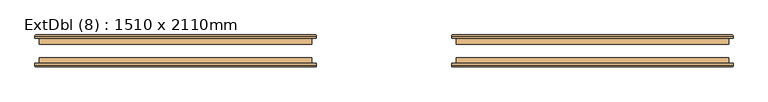
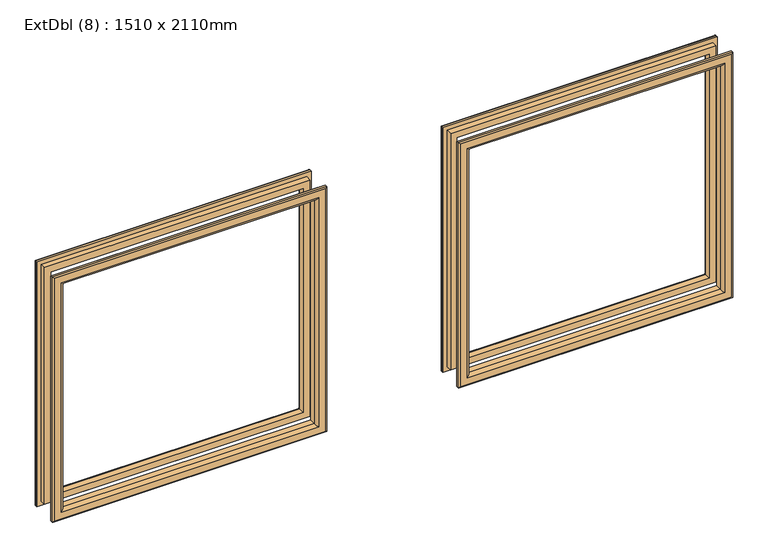
"""IFC4 building model written with IfcOpenShell, lengths in millimetres: door geometry, ExtDbl (8) : 1510 x 2110mm."""

from ifc_helpers import new_model, si_unit, frame, origin, place, context, project, spatial, ellipse_curve, source, transform, mapped, element, save
from ifc_brep_helpers import plane_surface, cylinder_surface, advanced_brep


def extdbl_8_1510_x_2110mm_bd11c51c(model_context):
    return source(origin(), model_context, "Body", "AdvancedBrep", [
        advanced_brep(
        [(-126.5, 31.0, 808.5), (-126.5, 21.0, 808.5), (-126.5, 21.0, 358.5), (-126.5, 31.0, 358.5), (-138.5, 20.0, 796.5), (-138.5, 31.0, 796.5), (-138.5, 31.0, 370.5), (-138.5, 20.0, 370.5), (-133.5, 15.0, 801.5), (-133.5, 15.0, 365.5), (-118.5, 17.0, 816.5), (-120.5, 15.0, 814.5), (-120.5, 15.0, 352.5), (-118.5, 17.0, 350.5), (-118.5, 21.0, 816.5), (-118.5, 21.0, 350.5), (-603.5, 21.0, 358.5), (-603.5, 31.0, 358.5), (-591.5, 31.0, 370.5), (-591.5, 20.0, 370.5), (-596.5, 15.0, 365.5), (-609.5, 15.0, 352.5), (-611.5, 17.0, 350.5), (-611.5, 21.0, 350.5), (-603.5, 21.0, 808.5), (-603.5, 31.0, 808.5), (-591.5, 31.0, 796.5), (-591.5, 20.0, 796.5), (-596.5, 15.0, 801.5), (-609.5, 15.0, 814.5), (-611.5, 17.0, 816.5), (-611.5, 21.0, 816.5)],
        [
            (0, 1),
            (1, 2),
            (2, 3),
            (3, 0),
            (4, 5),
            (5, 6),
            (6, 7),
            (7, 4),
            (8, 4, ellipse_curve(frame((-133.5, 20.0, 801.5), z_axis=(0.707106781186552, 0.0, -0.7071067811865429), x_axis=(0.7071067811865428, 0.0, 0.7071067811865521)), 7.0710678, 5.0)),
            (7, 9, ellipse_curve(frame((-133.5, 20.0, 365.5), z_axis=(0.7071067811865429, 0.0, 0.707106781186552), x_axis=(-0.707106781186552, 0.0, 0.707106781186543)), 7.0710678, 5.0)),
            (9, 8),
            (10, 11, ellipse_curve(frame((-120.5, 17.0, 814.5), z_axis=(0.707106781186552, 0.0, -0.7071067811865429), x_axis=(0.7071067811865428, 0.0, 0.7071067811865521)), 2.8284271, 2.0)),
            (11, 12),
            (12, 13, ellipse_curve(frame((-120.5, 17.0, 352.5), z_axis=(0.7071067811865429, 0.0, 0.707106781186552), x_axis=(-0.707106781186552, 0.0, 0.707106781186543)), 2.8284271, 2.0)),
            (13, 10),
            (14, 10),
            (13, 15),
            (15, 14),
            (2, 16),
            (16, 17),
            (17, 3),
            (6, 18),
            (18, 19),
            (19, 7),
            (19, 20, ellipse_curve(frame((-596.5, 20.0, 365.5), z_axis=(0.7071067811865521, 0.0, -0.7071067811865428), x_axis=(0.7071067811865429, 0.0, 0.707106781186552)), 7.0710678, 5.0)),
            (20, 9),
            (12, 21),
            (21, 22, ellipse_curve(frame((-609.5, 17.0, 352.5), z_axis=(0.7071067811865521, 0.0, -0.7071067811865428), x_axis=(0.7071067811865429, 0.0, 0.707106781186552)), 2.8284271, 2.0)),
            (22, 13),
            (22, 23),
            (23, 15),
            (16, 24),
            (24, 25),
            (25, 17),
            (18, 26),
            (26, 27),
            (27, 19),
            (27, 28, ellipse_curve(frame((-596.5, 20.0, 801.5), z_axis=(-0.7071067811865428, 0.0, -0.7071067811865521), x_axis=(0.707106781186552, 0.0, -0.7071067811865429)), 7.0710678, 5.0)),
            (28, 20),
            (21, 29),
            (29, 30, ellipse_curve(frame((-609.5, 17.0, 814.5), z_axis=(-0.7071067811865428, 0.0, -0.7071067811865521), x_axis=(0.707106781186552, 0.0, -0.7071067811865429)), 2.8284271, 2.0)),
            (30, 22),
            (30, 31),
            (31, 23),
            (31, 14),
            (1, 24),
            (0, 25),
            (5, 26),
            (4, 27),
            (8, 28),
            (11, 29),
            (10, 30),
        ],
        [
            plane_surface(frame((-126.5, 21.0, 808.5), z_axis=(1.0, 0.0, 0.0), x_axis=(0.0, 0.0, -1.0))),
            plane_surface(frame((-138.5, 31.0, 796.5), z_axis=(-1.0, 0.0, 0.0), x_axis=(0.0, 0.0, -1.0))),
            cylinder_surface(frame((-133.5, 20.0, 808.5), z_axis=(0.0, 0.0, 1.0), x_axis=(1.0, 0.0, 0.0)), 5.0),
            cylinder_surface(frame((-120.5, 17.0, 808.5), z_axis=(0.0, 0.0, 1.0), x_axis=(1.0, 0.0, 0.0)), 2.0),
            plane_surface(frame((-118.5, 17.0, 816.5), z_axis=(1.0, 0.0, 0.0), x_axis=(0.0, 0.0, -1.0))),
            plane_surface(frame((-126.5, 21.0, 358.5), z_axis=(0.0, 0.0, -1.0), x_axis=(-1.0, 0.0, 0.0))),
            plane_surface(frame((-138.5, 31.0, 370.5), z_axis=(0.0, 0.0, 1.0), x_axis=(-1.0, 0.0, 0.0))),
            cylinder_surface(frame((-126.5, 20.0, 365.5), z_axis=(1.0, 0.0, 0.0), x_axis=(0.0, 0.0, -1.0)), 5.0),
            cylinder_surface(frame((-126.5, 17.0, 352.5), z_axis=(1.0, 0.0, 0.0), x_axis=(0.0, 0.0, -1.0)), 2.0),
            plane_surface(frame((-118.5, 17.0, 350.5), z_axis=(0.0, 0.0, -1.0), x_axis=(-1.0, 0.0, 0.0))),
            plane_surface(frame((-603.5, 21.0, 358.5), z_axis=(-1.0, 0.0, 0.0), x_axis=(0.0, 0.0, 1.0))),
            plane_surface(frame((-591.5, 31.0, 370.5), z_axis=(1.0, 0.0, 0.0), x_axis=(0.0, 0.0, 1.0))),
            cylinder_surface(frame((-596.5, 20.0, 358.5), z_axis=(0.0, 0.0, -1.0), x_axis=(-1.0, 0.0, 0.0)), 5.0),
            cylinder_surface(frame((-609.5, 17.0, 358.5), z_axis=(0.0, 0.0, -1.0), x_axis=(-1.0, 0.0, 0.0)), 2.0),
            plane_surface(frame((-611.5, 17.0, 350.5), z_axis=(-1.0, 0.0, 0.0), x_axis=(0.0, 0.0, 1.0))),
            plane_surface(frame((-611.5, 21.0, 816.5), z_axis=(0.0, 1.0, 0.0), x_axis=(1.0, 0.0, 0.0))),
            plane_surface(frame((-603.5, 21.0, 808.5), z_axis=(0.0, 0.0, 1.0), x_axis=(1.0, 0.0, 0.0))),
            plane_surface(frame((-603.5, 31.0, 808.5), z_axis=(0.0, 1.0, 0.0), x_axis=(1.0, 0.0, 0.0))),
            plane_surface(frame((-591.5, 31.0, 796.5), z_axis=(0.0, 0.0, -1.0), x_axis=(1.0, 0.0, 0.0))),
            cylinder_surface(frame((-603.5, 20.0, 801.5), z_axis=(-1.0, 0.0, 0.0), x_axis=(0.0, 0.0, 1.0)), 5.0),
            plane_surface(frame((-596.5, 15.0, 801.5), z_axis=(0.0, -1.0, 0.0), x_axis=(1.0, 0.0, 0.0))),
            cylinder_surface(frame((-603.5, 17.0, 814.5), z_axis=(-1.0, 0.0, 0.0), x_axis=(0.0, 0.0, 1.0)), 2.0),
            plane_surface(frame((-611.5, 17.0, 816.5), z_axis=(0.0, 0.0, 1.0), x_axis=(1.0, 0.0, 0.0))),
        ],
        [
            (0, [[1, 2, 3, 4]]),
            (1, [[5, 6, 7, 8]]),
            (2, [[9, -8, 10, 11]]),
            (3, [[12, 13, 14, 15]]),
            (4, [[16, -15, 17, 18]]),
            (5, [[-3, 19, 20, 21]]),
            (6, [[-7, 22, 23, 24]]),
            (7, [[-10, -24, 25, 26]]),
            (8, [[-14, 27, 28, 29]]),
            (9, [[-17, -29, 30, 31]]),
            (10, [[-20, 32, 33, 34]]),
            (11, [[-23, 35, 36, 37]]),
            (12, [[-25, -37, 38, 39]]),
            (13, [[-28, 40, 41, 42]]),
            (14, [[-30, -42, 43, 44]]),
            (15, [[-31, -44, 45, -18], [46, -32, -19, -2]]),
            (16, [[-33, -46, -1, 47]]),
            (17, [[-21, -34, -47, -4], [48, -35, -22, -6]]),
            (18, [[-36, -48, -5, 49]]),
            (19, [[-38, -49, -9, 50]]),
            (20, [[51, -40, -27, -13], [-26, -39, -50, -11]]),
            (21, [[-41, -51, -12, 52]]),
            (22, [[-43, -52, -16, -45]]),
        ],
    ),
        advanced_brep(
        [(-603.5, 55.0, 808.5), (-603.5, 65.0, 808.5), (-603.5, 65.0, 358.5), (-603.5, 55.0, 358.5), (-591.5, 66.0, 796.5), (-591.5, 55.0, 796.5), (-591.5, 55.0, 370.5), (-591.5, 66.0, 370.5), (-596.5, 71.0, 801.5), (-596.5, 71.0, 365.5), (-611.5, 69.0, 816.5), (-609.5, 71.0, 814.5), (-609.5, 71.0, 352.5), (-611.5, 69.0, 350.5), (-611.5, 65.0, 816.5), (-611.5, 65.0, 350.5), (-126.5, 65.0, 358.5), (-126.5, 55.0, 358.5), (-138.5, 55.0, 370.5), (-138.5, 66.0, 370.5), (-133.5, 71.0, 365.5), (-120.5, 71.0, 352.5), (-118.5, 69.0, 350.5), (-118.5, 65.0, 350.5), (-126.5, 65.0, 808.5), (-126.5, 55.0, 808.5), (-138.5, 55.0, 796.5), (-138.5, 66.0, 796.5), (-133.5, 71.0, 801.5), (-120.5, 71.0, 814.5), (-118.5, 69.0, 816.5), (-118.5, 65.0, 816.5)],
        [
            (0, 1),
            (1, 2),
            (2, 3),
            (3, 0),
            (4, 5),
            (5, 6),
            (6, 7),
            (7, 4),
            (8, 4, ellipse_curve(frame((-596.5, 66.0, 801.5), z_axis=(-0.7071067811865477, 0.0, -0.7071067811865472), x_axis=(-0.7071067811865471, 0.0, 0.7071067811865478)), 7.0710678, 5.0)),
            (7, 9, ellipse_curve(frame((-596.5, 66.0, 365.5), z_axis=(-0.7071067811865472, 0.0, 0.7071067811865477), x_axis=(0.7071067811865476, 0.0, 0.7071067811865475)), 7.0710678, 5.0)),
            (9, 8),
            (10, 11, ellipse_curve(frame((-609.5, 69.0, 814.5), z_axis=(-0.7071067811865477, 0.0, -0.7071067811865472), x_axis=(-0.7071067811865471, 0.0, 0.7071067811865478)), 2.8284271, 2.0)),
            (11, 12),
            (12, 13, ellipse_curve(frame((-609.5, 69.0, 352.5), z_axis=(-0.7071067811865472, 0.0, 0.7071067811865477), x_axis=(0.7071067811865476, 0.0, 0.7071067811865475)), 2.8284271, 2.0)),
            (13, 10),
            (14, 10),
            (13, 15),
            (15, 14),
            (2, 16),
            (16, 17),
            (17, 3),
            (6, 18),
            (18, 19),
            (19, 7),
            (19, 20, ellipse_curve(frame((-133.5, 66.0, 365.5), z_axis=(-0.7071067811865477, 0.0, -0.7071067811865474), x_axis=(-0.7071067811865474, 0.0, 0.7071067811865478)), 7.0710678, 5.0)),
            (20, 9),
            (12, 21),
            (21, 22, ellipse_curve(frame((-120.5, 69.0, 352.5), z_axis=(-0.7071067811865477, 0.0, -0.7071067811865474), x_axis=(-0.7071067811865474, 0.0, 0.7071067811865478)), 2.8284271, 2.0)),
            (22, 13),
            (22, 23),
            (23, 15),
            (16, 24),
            (24, 25),
            (25, 17),
            (18, 26),
            (26, 27),
            (27, 19),
            (27, 28, ellipse_curve(frame((-133.5, 66.0, 801.5), z_axis=(0.7071067811865474, 0.0, -0.7071067811865478), x_axis=(-0.7071067811865479, 0.0, -0.7071067811865471)), 7.0710678, 5.0)),
            (28, 20),
            (21, 29),
            (29, 30, ellipse_curve(frame((-120.5, 69.0, 814.5), z_axis=(0.7071067811865474, 0.0, -0.7071067811865478), x_axis=(-0.7071067811865479, 0.0, -0.7071067811865471)), 2.8284271, 2.0)),
            (30, 22),
            (30, 31),
            (31, 23),
            (31, 14),
            (1, 24),
            (0, 25),
            (5, 26),
            (4, 27),
            (8, 28),
            (11, 29),
            (10, 30),
        ],
        [
            plane_surface(frame((-603.5, 65.0, 808.5), z_axis=(-1.0, 0.0, 0.0), x_axis=(0.0, 0.0, -1.0))),
            plane_surface(frame((-591.5, 55.0, 796.5), z_axis=(1.0, 0.0, 0.0), x_axis=(0.0, 0.0, -1.0))),
            cylinder_surface(frame((-596.5, 66.0, 808.5), z_axis=(0.0, 0.0, 1.0), x_axis=(-1.0, 0.0, 0.0)), 5.0),
            cylinder_surface(frame((-609.5, 69.0, 808.5), z_axis=(0.0, 0.0, 1.0), x_axis=(-1.0, 0.0, 0.0)), 2.0),
            plane_surface(frame((-611.5, 69.0, 816.5), z_axis=(-1.0, 0.0, 0.0), x_axis=(0.0, 0.0, -1.0))),
            plane_surface(frame((-603.5, 65.0, 358.5), z_axis=(0.0, 0.0, -1.0), x_axis=(1.0, 0.0, 0.0))),
            plane_surface(frame((-591.5, 55.0, 370.5), z_axis=(0.0, 0.0, 1.0), x_axis=(1.0, 0.0, 0.0))),
            cylinder_surface(frame((-603.5, 66.0, 365.5), z_axis=(-1.0, 0.0, 0.0), x_axis=(0.0, 0.0, -1.0)), 5.0),
            cylinder_surface(frame((-603.5, 69.0, 352.5), z_axis=(-1.0, 0.0, 0.0), x_axis=(0.0, 0.0, -1.0)), 2.0),
            plane_surface(frame((-611.5, 69.0, 350.5), z_axis=(0.0, 0.0, -1.0), x_axis=(1.0, 0.0, 0.0))),
            plane_surface(frame((-126.5, 65.0, 358.5), z_axis=(1.0, 0.0, 0.0), x_axis=(0.0, 0.0, 1.0))),
            plane_surface(frame((-138.5, 55.0, 370.5), z_axis=(-1.0, 0.0, 0.0), x_axis=(0.0, 0.0, 1.0))),
            cylinder_surface(frame((-133.5, 66.0, 358.5), z_axis=(0.0, 0.0, -1.0), x_axis=(1.0, 0.0, 0.0)), 5.0),
            cylinder_surface(frame((-120.5, 69.0, 358.5), z_axis=(0.0, 0.0, -1.0), x_axis=(1.0, 0.0, 0.0)), 2.0),
            plane_surface(frame((-118.5, 69.0, 350.5), z_axis=(1.0, 0.0, 0.0), x_axis=(0.0, 0.0, 1.0))),
            plane_surface(frame((-118.5, 65.0, 816.5), z_axis=(0.0, -1.0, 0.0), x_axis=(-1.0, 0.0, 0.0))),
            plane_surface(frame((-126.5, 65.0, 808.5), z_axis=(0.0, 0.0, 1.0), x_axis=(-1.0, 0.0, 0.0))),
            plane_surface(frame((-126.5, 55.0, 808.5), z_axis=(0.0, -1.0, 0.0), x_axis=(-1.0, 0.0, 0.0))),
            plane_surface(frame((-138.5, 55.0, 796.5), z_axis=(0.0, 0.0, -1.0), x_axis=(-1.0, 0.0, 0.0))),
            cylinder_surface(frame((-126.5, 66.0, 801.5), z_axis=(1.0, 0.0, 0.0), x_axis=(0.0, 0.0, 1.0)), 5.0),
            plane_surface(frame((-133.5, 71.0, 801.5), z_axis=(0.0, 1.0, 0.0), x_axis=(-1.0, 0.0, 0.0))),
            cylinder_surface(frame((-126.5, 69.0, 814.5), z_axis=(1.0, 0.0, 0.0), x_axis=(0.0, 0.0, 1.0)), 2.0),
            plane_surface(frame((-118.5, 69.0, 816.5), z_axis=(0.0, 0.0, 1.0), x_axis=(-1.0, 0.0, 0.0))),
        ],
        [
            (0, [[1, 2, 3, 4]]),
            (1, [[5, 6, 7, 8]]),
            (2, [[9, -8, 10, 11]]),
            (3, [[12, 13, 14, 15]]),
            (4, [[16, -15, 17, 18]]),
            (5, [[-3, 19, 20, 21]]),
            (6, [[-7, 22, 23, 24]]),
            (7, [[-10, -24, 25, 26]]),
            (8, [[-14, 27, 28, 29]]),
            (9, [[-17, -29, 30, 31]]),
            (10, [[-20, 32, 33, 34]]),
            (11, [[-23, 35, 36, 37]]),
            (12, [[-25, -37, 38, 39]]),
            (13, [[-28, 40, 41, 42]]),
            (14, [[-30, -42, 43, 44]]),
            (15, [[-31, -44, 45, -18], [46, -32, -19, -2]]),
            (16, [[-33, -46, -1, 47]]),
            (17, [[-21, -34, -47, -4], [48, -35, -22, -6]]),
            (18, [[-36, -48, -5, 49]]),
            (19, [[-38, -49, -9, 50]]),
            (20, [[51, -40, -27, -13], [-26, -39, -50, -11]]),
            (21, [[-41, -51, -12, 52]]),
            (22, [[-43, -52, -16, -45]]),
        ],
    ),
        advanced_brep(
        [(603.5, 31.0, 808.5), (603.5, 21.0, 808.5), (603.5, 21.0, 358.5), (603.5, 31.0, 358.5), (591.5, 20.0, 796.5), (591.5, 31.0, 796.5), (591.5, 31.0, 370.5), (591.5, 20.0, 370.5), (596.5, 15.0, 801.5), (596.5, 15.0, 365.5), (611.5, 17.0, 816.5), (609.5, 15.0, 814.5), (609.5, 15.0, 352.5), (611.5, 17.0, 350.5), (611.5, 21.0, 816.5), (611.5, 21.0, 350.5), (126.5, 21.0, 358.5), (126.5, 31.0, 358.5), (138.5, 31.0, 370.5), (138.5, 20.0, 370.5), (133.5, 15.0, 365.5), (120.5, 15.0, 352.5), (118.5, 17.0, 350.5), (118.5, 21.0, 350.5), (126.5, 21.0, 808.5), (126.5, 31.0, 808.5), (138.5, 31.0, 796.5), (138.5, 20.0, 796.5), (133.5, 15.0, 801.5), (120.5, 15.0, 814.5), (118.5, 17.0, 816.5), (118.5, 21.0, 816.5)],
        [
            (0, 1),
            (1, 2),
            (2, 3),
            (3, 0),
            (4, 5),
            (5, 6),
            (6, 7),
            (7, 4),
            (8, 4, ellipse_curve(frame((596.5, 20.0, 801.5), z_axis=(0.7071067811865519, 0.0, -0.707106781186543), x_axis=(0.7071067811865429, 0.0, 0.7071067811865521)), 7.0710678, 5.0)),
            (7, 9, ellipse_curve(frame((596.5, 20.0, 365.5), z_axis=(0.707106781186543, 0.0, 0.707106781186552), x_axis=(-0.707106781186552, 0.0, 0.707106781186543)), 7.0710678, 5.0)),
            (9, 8),
            (10, 11, ellipse_curve(frame((609.5, 17.0, 814.5), z_axis=(0.7071067811865519, 0.0, -0.707106781186543), x_axis=(0.7071067811865429, 0.0, 0.7071067811865521)), 2.8284271, 2.0)),
            (11, 12),
            (12, 13, ellipse_curve(frame((609.5, 17.0, 352.5), z_axis=(0.707106781186543, 0.0, 0.707106781186552), x_axis=(-0.707106781186552, 0.0, 0.707106781186543)), 2.8284271, 2.0)),
            (13, 10),
            (14, 10),
            (13, 15),
            (15, 14),
            (2, 16),
            (16, 17),
            (17, 3),
            (6, 18),
            (18, 19),
            (19, 7),
            (19, 20, ellipse_curve(frame((133.5, 20.0, 365.5), z_axis=(0.707106781186552, 0.0, -0.707106781186543), x_axis=(0.7071067811865429, 0.0, 0.707106781186552)), 7.0710678, 5.0)),
            (20, 9),
            (12, 21),
            (21, 22, ellipse_curve(frame((120.5, 17.0, 352.5), z_axis=(0.707106781186552, 0.0, -0.707106781186543), x_axis=(0.7071067811865429, 0.0, 0.707106781186552)), 2.8284271, 2.0)),
            (22, 13),
            (22, 23),
            (23, 15),
            (16, 24),
            (24, 25),
            (25, 17),
            (18, 26),
            (26, 27),
            (27, 19),
            (27, 28, ellipse_curve(frame((133.5, 20.0, 801.5), z_axis=(-0.7071067811865431, 0.0, -0.707106781186552), x_axis=(0.7071067811865521, 0.0, -0.7071067811865429)), 7.0710678, 5.0)),
            (28, 20),
            (21, 29),
            (29, 30, ellipse_curve(frame((120.5, 17.0, 814.5), z_axis=(-0.7071067811865431, 0.0, -0.707106781186552), x_axis=(0.7071067811865521, 0.0, -0.7071067811865429)), 2.8284271, 2.0)),
            (30, 22),
            (30, 31),
            (31, 23),
            (31, 14),
            (1, 24),
            (0, 25),
            (5, 26),
            (4, 27),
            (8, 28),
            (11, 29),
            (10, 30),
        ],
        [
            plane_surface(frame((603.5, 21.0, 808.5), z_axis=(1.0, 0.0, 0.0), x_axis=(0.0, 0.0, -1.0))),
            plane_surface(frame((591.5, 31.0, 796.5), z_axis=(-1.0, 0.0, 0.0), x_axis=(0.0, 0.0, -1.0))),
            cylinder_surface(frame((596.5, 20.0, 808.5), z_axis=(0.0, 0.0, 1.0), x_axis=(1.0, 0.0, 0.0)), 5.0),
            cylinder_surface(frame((609.5, 17.0, 808.5), z_axis=(0.0, 0.0, 1.0), x_axis=(1.0, 0.0, 0.0)), 2.0),
            plane_surface(frame((611.5, 17.0, 816.5), z_axis=(1.0, 0.0, 0.0), x_axis=(0.0, 0.0, -1.0))),
            plane_surface(frame((603.5, 21.0, 358.5), z_axis=(0.0, 0.0, -1.0), x_axis=(-1.0, 0.0, 0.0))),
            plane_surface(frame((591.5, 31.0, 370.5), z_axis=(0.0, 0.0, 1.0), x_axis=(-1.0, 0.0, 0.0))),
            cylinder_surface(frame((603.5, 20.0, 365.5), z_axis=(1.0, 0.0, 0.0), x_axis=(0.0, 0.0, -1.0)), 5.0),
            cylinder_surface(frame((603.5, 17.0, 352.5), z_axis=(1.0, 0.0, 0.0), x_axis=(0.0, 0.0, -1.0)), 2.0),
            plane_surface(frame((611.5, 17.0, 350.5), z_axis=(0.0, 0.0, -1.0), x_axis=(-1.0, 0.0, 0.0))),
            plane_surface(frame((126.5, 21.0, 358.5), z_axis=(-1.0, 0.0, 0.0), x_axis=(0.0, 0.0, 1.0))),
            plane_surface(frame((138.5, 31.0, 370.5), z_axis=(1.0, 0.0, 0.0), x_axis=(0.0, 0.0, 1.0))),
            cylinder_surface(frame((133.5, 20.0, 358.5), z_axis=(0.0, 0.0, -1.0), x_axis=(-1.0, 0.0, 0.0)), 5.0),
            cylinder_surface(frame((120.5, 17.0, 358.5), z_axis=(0.0, 0.0, -1.0), x_axis=(-1.0, 0.0, 0.0)), 2.0),
            plane_surface(frame((118.5, 17.0, 350.5), z_axis=(-1.0, 0.0, 0.0), x_axis=(0.0, 0.0, 1.0))),
            plane_surface(frame((118.5, 21.0, 816.5), z_axis=(0.0, 1.0, 0.0), x_axis=(1.0, 0.0, 0.0))),
            plane_surface(frame((126.5, 21.0, 808.5), z_axis=(0.0, 0.0, 1.0), x_axis=(1.0, 0.0, 0.0))),
            plane_surface(frame((126.5, 31.0, 808.5), z_axis=(0.0, 1.0, 0.0), x_axis=(1.0, 0.0, 0.0))),
            plane_surface(frame((138.5, 31.0, 796.5), z_axis=(0.0, 0.0, -1.0), x_axis=(1.0, 0.0, 0.0))),
            cylinder_surface(frame((126.5, 20.0, 801.5), z_axis=(-1.0, 0.0, 0.0), x_axis=(0.0, 0.0, 1.0)), 5.0),
            plane_surface(frame((133.5, 15.0, 801.5), z_axis=(0.0, -1.0, 0.0), x_axis=(1.0, 0.0, 0.0))),
            cylinder_surface(frame((126.5, 17.0, 814.5), z_axis=(-1.0, 0.0, 0.0), x_axis=(0.0, 0.0, 1.0)), 2.0),
            plane_surface(frame((118.5, 17.0, 816.5), z_axis=(0.0, 0.0, 1.0), x_axis=(1.0, 0.0, 0.0))),
        ],
        [
            (0, [[1, 2, 3, 4]]),
            (1, [[5, 6, 7, 8]]),
            (2, [[9, -8, 10, 11]]),
            (3, [[12, 13, 14, 15]]),
            (4, [[16, -15, 17, 18]]),
            (5, [[-3, 19, 20, 21]]),
            (6, [[-7, 22, 23, 24]]),
            (7, [[-10, -24, 25, 26]]),
            (8, [[-14, 27, 28, 29]]),
            (9, [[-17, -29, 30, 31]]),
            (10, [[-20, 32, 33, 34]]),
            (11, [[-23, 35, 36, 37]]),
            (12, [[-25, -37, 38, 39]]),
            (13, [[-28, 40, 41, 42]]),
            (14, [[-30, -42, 43, 44]]),
            (15, [[-31, -44, 45, -18], [46, -32, -19, -2]]),
            (16, [[-33, -46, -1, 47]]),
            (17, [[-21, -34, -47, -4], [48, -35, -22, -6]]),
            (18, [[-36, -48, -5, 49]]),
            (19, [[-38, -49, -9, 50]]),
            (20, [[51, -40, -27, -13], [-26, -39, -50, -11]]),
            (21, [[-41, -51, -12, 52]]),
            (22, [[-43, -52, -16, -45]]),
        ],
    ),
        advanced_brep(
        [(126.5, 55.0, 808.5), (126.5, 65.0, 808.5), (126.5, 65.0, 358.5), (126.5, 55.0, 358.5), (138.5, 66.0, 796.5), (138.5, 55.0, 796.5), (138.5, 55.0, 370.5), (138.5, 66.0, 370.5), (133.5, 71.0, 801.5), (133.5, 71.0, 365.5), (118.5, 69.0, 816.5), (120.5, 71.0, 814.5), (120.5, 71.0, 352.5), (118.5, 69.0, 350.5), (118.5, 65.0, 816.5), (118.5, 65.0, 350.5), (603.5, 65.0, 358.5), (603.5, 55.0, 358.5), (591.5, 55.0, 370.5), (591.5, 66.0, 370.5), (596.5, 71.0, 365.5), (609.5, 71.0, 352.5), (611.5, 69.0, 350.5), (611.5, 65.0, 350.5), (603.5, 65.0, 808.5), (603.5, 55.0, 808.5), (591.5, 55.0, 796.5), (591.5, 66.0, 796.5), (596.5, 71.0, 801.5), (609.5, 71.0, 814.5), (611.5, 69.0, 816.5), (611.5, 65.0, 816.5)],
        [
            (0, 1),
            (1, 2),
            (2, 3),
            (3, 0),
            (4, 5),
            (5, 6),
            (6, 7),
            (7, 4),
            (8, 4, ellipse_curve(frame((133.5, 66.0, 801.5), z_axis=(-0.7071067811865475, 0.0, -0.7071067811865475), x_axis=(-0.7071067811865474, 0.0, 0.7071067811865476)), 7.0710678, 5.0)),
            (7, 9, ellipse_curve(frame((133.5, 66.0, 365.5), z_axis=(-0.7071067811865475, 0.0, 0.7071067811865475), x_axis=(0.7071067811865474, 0.0, 0.7071067811865476)), 7.0710678, 5.0)),
            (9, 8),
            (10, 11, ellipse_curve(frame((120.5, 69.0, 814.5), z_axis=(-0.7071067811865475, 0.0, -0.7071067811865475), x_axis=(-0.7071067811865474, 0.0, 0.7071067811865476)), 2.8284271, 2.0)),
            (11, 12),
            (12, 13, ellipse_curve(frame((120.5, 69.0, 352.5), z_axis=(-0.7071067811865475, 0.0, 0.7071067811865475), x_axis=(0.7071067811865474, 0.0, 0.7071067811865476)), 2.8284271, 2.0)),
            (13, 10),
            (14, 10),
            (13, 15),
            (15, 14),
            (2, 16),
            (16, 17),
            (17, 3),
            (6, 18),
            (18, 19),
            (19, 7),
            (19, 20, ellipse_curve(frame((596.5, 66.0, 365.5), z_axis=(-0.7071067811865475, 0.0, -0.7071067811865475), x_axis=(-0.7071067811865476, 0.0, 0.7071067811865474)), 7.0710678, 5.0)),
            (20, 9),
            (12, 21),
            (21, 22, ellipse_curve(frame((609.5, 69.0, 352.5), z_axis=(-0.7071067811865475, 0.0, -0.7071067811865475), x_axis=(-0.7071067811865476, 0.0, 0.7071067811865474)), 2.8284271, 2.0)),
            (22, 13),
            (22, 23),
            (23, 15),
            (16, 24),
            (24, 25),
            (25, 17),
            (18, 26),
            (26, 27),
            (27, 19),
            (27, 28, ellipse_curve(frame((596.5, 66.0, 801.5), z_axis=(0.7071067811865475, 0.0, -0.7071067811865475), x_axis=(-0.7071067811865474, 0.0, -0.7071067811865476)), 7.0710678, 5.0)),
            (28, 20),
            (21, 29),
            (29, 30, ellipse_curve(frame((609.5, 69.0, 814.5), z_axis=(0.7071067811865475, 0.0, -0.7071067811865475), x_axis=(-0.7071067811865474, 0.0, -0.7071067811865476)), 2.8284271, 2.0)),
            (30, 22),
            (30, 31),
            (31, 23),
            (31, 14),
            (1, 24),
            (0, 25),
            (5, 26),
            (4, 27),
            (8, 28),
            (11, 29),
            (10, 30),
        ],
        [
            plane_surface(frame((126.5, 65.0, 808.5), z_axis=(-1.0, 0.0, 0.0), x_axis=(0.0, 0.0, -1.0))),
            plane_surface(frame((138.5, 55.0, 796.5), z_axis=(1.0, 0.0, 0.0), x_axis=(0.0, 0.0, -1.0))),
            cylinder_surface(frame((133.5, 66.0, 808.5), z_axis=(0.0, 0.0, 1.0), x_axis=(-1.0, 0.0, 0.0)), 5.0),
            cylinder_surface(frame((120.5, 69.0, 808.5), z_axis=(0.0, 0.0, 1.0), x_axis=(-1.0, 0.0, 0.0)), 2.0),
            plane_surface(frame((118.5, 69.0, 816.5), z_axis=(-1.0, 0.0, 0.0), x_axis=(0.0, 0.0, -1.0))),
            plane_surface(frame((126.5, 65.0, 358.5), z_axis=(0.0, 0.0, -1.0), x_axis=(1.0, 0.0, 0.0))),
            plane_surface(frame((138.5, 55.0, 370.5), z_axis=(0.0, 0.0, 1.0), x_axis=(1.0, 0.0, 0.0))),
            cylinder_surface(frame((126.5, 66.0, 365.5), z_axis=(-1.0, 0.0, 0.0), x_axis=(0.0, 0.0, -1.0)), 5.0),
            cylinder_surface(frame((126.5, 69.0, 352.5), z_axis=(-1.0, 0.0, 0.0), x_axis=(0.0, 0.0, -1.0)), 2.0),
            plane_surface(frame((118.5, 69.0, 350.5), z_axis=(0.0, 0.0, -1.0), x_axis=(1.0, 0.0, 0.0))),
            plane_surface(frame((603.5, 65.0, 358.5), z_axis=(1.0, 0.0, 0.0), x_axis=(0.0, 0.0, 1.0))),
            plane_surface(frame((591.5, 55.0, 370.5), z_axis=(-1.0, 0.0, 0.0), x_axis=(0.0, 0.0, 1.0))),
            cylinder_surface(frame((596.5, 66.0, 358.5), z_axis=(0.0, 0.0, -1.0), x_axis=(1.0, 0.0, 0.0)), 5.0),
            cylinder_surface(frame((609.5, 69.0, 358.5), z_axis=(0.0, 0.0, -1.0), x_axis=(1.0, 0.0, 0.0)), 2.0),
            plane_surface(frame((611.5, 69.0, 350.5), z_axis=(1.0, 0.0, 0.0), x_axis=(0.0, 0.0, 1.0))),
            plane_surface(frame((611.5, 65.0, 816.5), z_axis=(0.0, -1.0, 0.0), x_axis=(-1.0, 0.0, 0.0))),
            plane_surface(frame((603.5, 65.0, 808.5), z_axis=(0.0, 0.0, 1.0), x_axis=(-1.0, 0.0, 0.0))),
            plane_surface(frame((603.5, 55.0, 808.5), z_axis=(0.0, -1.0, 0.0), x_axis=(-1.0, 0.0, 0.0))),
            plane_surface(frame((591.5, 55.0, 796.5), z_axis=(0.0, 0.0, -1.0), x_axis=(-1.0, 0.0, 0.0))),
            cylinder_surface(frame((603.5, 66.0, 801.5), z_axis=(1.0, 0.0, 0.0), x_axis=(0.0, 0.0, 1.0)), 5.0),
            plane_surface(frame((596.5, 71.0, 801.5), z_axis=(0.0, 1.0, 0.0), x_axis=(-1.0, 0.0, 0.0))),
            cylinder_surface(frame((603.5, 69.0, 814.5), z_axis=(1.0, 0.0, 0.0), x_axis=(0.0, 0.0, 1.0)), 2.0),
            plane_surface(frame((611.5, 69.0, 816.5), z_axis=(0.0, 0.0, 1.0), x_axis=(-1.0, 0.0, 0.0))),
        ],
        [
            (0, [[1, 2, 3, 4]]),
            (1, [[5, 6, 7, 8]]),
            (2, [[9, -8, 10, 11]]),
            (3, [[12, 13, 14, 15]]),
            (4, [[16, -15, 17, 18]]),
            (5, [[-3, 19, 20, 21]]),
            (6, [[-7, 22, 23, 24]]),
            (7, [[-10, -24, 25, 26]]),
            (8, [[-14, 27, 28, 29]]),
            (9, [[-17, -29, 30, 31]]),
            (10, [[-20, 32, 33, 34]]),
            (11, [[-23, 35, 36, 37]]),
            (12, [[-25, -37, 38, 39]]),
            (13, [[-28, 40, 41, 42]]),
            (14, [[-30, -42, 43, 44]]),
            (15, [[-31, -44, 45, -18], [46, -32, -19, -2]]),
            (16, [[-33, -46, -1, 47]]),
            (17, [[-21, -34, -47, -4], [48, -35, -22, -6]]),
            (18, [[-36, -48, -5, 49]]),
            (19, [[-38, -49, -9, 50]]),
            (20, [[51, -40, -27, -13], [-26, -39, -50, -11]]),
            (21, [[-41, -51, -12, 52]]),
            (22, [[-43, -52, -16, -45]]),
        ],
    ),
    ])


if __name__ == "__main__":
    model = new_model("IFC4")
    model_context = context("Model", 3, world=origin())
    ifc_project = project(units=[si_unit("LENGTHUNIT", "METRE", prefix="MILLI")], contexts=[model_context])
    site = spatial("IfcSite", under=ifc_project)
    building = spatial("IfcBuilding", under=site)
    placement = place(None, origin())
    extdbl_8_1510_x_2110mm_shape = extdbl_8_1510_x_2110mm_bd11c51c(model_context)
    element("IfcDoor", 1, ObjectType="ExtDbl (8) : 1510 x 2110mm", at=placement, inside=building, context=model_context, shape_type="MappedRepresentation", body=[
        mapped(extdbl_8_1510_x_2110mm_shape, transform((0.0, 0.0, 0.0), x_axis=(1.0, 0.0, 0.0), y_axis=(0.0, 1.0, 0.0), z_axis=(0.0, 0.0, 1.0))),
    ])
    save(model, "model.ifc")

# Revit data of these elements
# Type "ExtDbl (8) : 1510 x 2110mm"
#   Type Mark = "13"
#   Type Comments = "External Double"
#   Operation = "DoubleDoorSingleSwing"
#   Keynote = "L20"
#   Wrap Layers (Int) from Ext = 177.5 mm
#   Wrap Layers (Ext) from Ext = 102.5 mm
#   Top of Lock Rail = 900 mm
#   Thickness = 44 mm
#   Stile Shutting = 125 mm
#   Stile - Top Rail = 150 mm
#   Stile - Lock Rail = 150 mm
#   Stile - Hanging = 100 mm
#   Stile - Bottom Rail = 300 mm
#   Rough Width = 1510 mm
#   Rough Height = 2110 mm
#   O/A Frame Width = 64 mm
#   Handle Z Distance = 950 mm
#   Glazing Thickness = 24 mm
#   FrameWidth = 42 mm
#   FrameOffset - External = 65 mm
#   FrameDepth = 89 mm
#   Door Panel Width = 702 mm
#   Door Panel Thickness = 44 mm
#   Door Panel Height = 2000 mm
#   Cill Thickness = 54.5 mm
#   Cill Projection = 30 mm
#   Handle X Distance = 75 mm
#   Height = 2110 mm
#   Structural Tolerance = 6.5 mm
#   Tolerance = 3 mm
#   Undercut = 4 mm
#   Width = 1510 mm
#   Cill Extension = 25 mm
#   Cavity Closer Width = 50 mm
#   Cavity Closer Offset from Ext = 102.5 mm
#   Cavity Closer Depth = 85 mm
#   Vis - Ironmongery = yes
#   Vis - Cavity Closers = yes
#   Function = 1
#   Material Glass = Door - Glazing
#   Handle Style = element 171650
#   Material Door = Door - Panel
#   Material Frame = Door - Frame/Mullion
#   Material Ironmongery = Door - Handle
#   Wall Closure = (empty or 0)
# Element 1 (IfcDoor, "ExtDbl (8) : 1510 x 2110mm")
#   Materials on its faces: "Door - Panel", "Door - Handle", "Door - Frame/Mullion", "Door - Glazing"
# Materials
#   "Door - Glazing": class "Miscellaneous", colour RGB 0 0 255, transparency 0.75
#   "Door - Panel": class "Wood", colour RGB 210 159 95, transparency 0
#   "Door - Frame/Mullion": class "Wood", colour RGB 212 179 113, transparency 0
#   "Door - Handle": class "Miscellaneous", colour RGB 247 247 247, transparency 0
